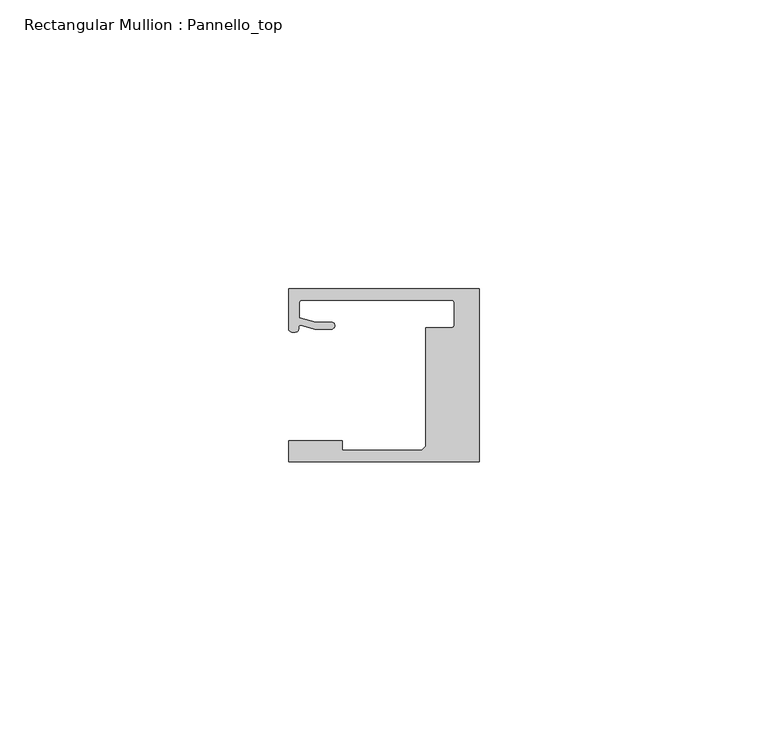
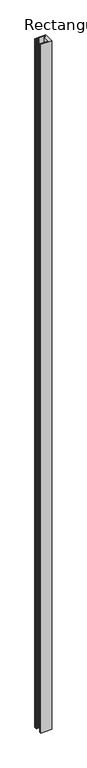
"""IFC4 building model written with IfcOpenShell, lengths in millimetres: member geometry, Rectangular Mullion : Pannello_top."""

from ifc_helpers import new_model, si_unit, frame, origin, place, context, project, spatial, polyline, circle_curve, source, transform, mapped, element, save
from ifc_brep_helpers import plane_surface, cylinder_surface, revolved_surface, extruded_surface, spline_curve, advanced_brep


def rectangular_mullion_pannello_top_90c1ebb8(model_context):
    return source(origin(), model_context, "Body", "AdvancedBrep", [
        advanced_brep(
        [(-33.0, -15.0, 0.0), (0.0, -15.0, 0.0), (0.0, 15.0, 0.0), (-33.0000135, 15.0, 0.0), (-33.0000135, 8.0000472, 0.0), (-30.9223017, 8.6490241, 0.0), (-28.4999305, 7.9999523, 0.0), (-25.59998, 7.9999523, 0.0), (-25.59998, 9.1999523, 0.0), (-28.3419477, 9.1999523, 0.0), (-31.19998, 9.9657591, 0.0), (-31.19998, 12.50001, 0.0), (-30.69998, 13.00001, 0.0), (-4.7999726, 13.00001, 0.0), (-4.2999726, 12.50001, 0.0), (-4.2999726, 8.7500595, 0.0), (-4.7999726, 8.2500595, 0.0), (-9.2999726, 8.2500595, 0.0), (-9.2999726, -12.2999849, 0.0), (-10.0000103, -13.0000004, 0.0), (-23.700041, -13.0000004, 0.0), (-23.700041, -11.3000004, 0.0), (-33.0, -11.3000004, 0.0), (-33.0, -15.0, -2173.9999729), (-33.0, -11.3000004, -2173.9999729), (-23.700041, -11.3000004, -2173.9999729), (-23.700041, -13.0000004, -2173.9999729), (-10.0000103, -13.0000004, -2173.9999729), (-9.2999726, -12.2999849, -2173.9999729), (-9.2999726, 8.2500595, -2173.9999729), (-4.7999726, 8.2500595, -2173.9999729), (-4.2999726, 8.7500595, -2173.9999729), (-4.2999726, 12.50001, -2173.9999729), (-4.7999726, 13.00001, -2173.9999729), (-30.69998, 13.00001, -2173.9999729), (-31.19998, 12.50001, -2173.9999729), (-31.19998, 9.9657591, -2173.9999729), (-28.3419477, 9.1999523, -2173.9999729), (-25.59998, 9.1999523, -2173.9999729), (-25.59998, 7.9999523, -2173.9999729), (-28.4999305, 7.9999523, -2173.9999729), (-30.9223017, 8.6490241, -2173.9999729), (-33.0000135, 8.0000472, -2173.9999729), (-33.0000135, 15.0, -2173.9999729), (0.0, 15.0, -2173.9999729), (0.0, -15.0, -2173.9999729)],
        [
            (0, 1),
            (1, 2),
            (2, 3),
            (3, 4),
            (4, 5, spline_curve(3, [(-33.0000135, 8.0000472, 0.0), (-33.0000135, 7.457047519, 0.0), (-32.262327879, 7.456527435, 0.0), (-31.357433266, 7.563996614, 0.0), (-31.305645054, 7.690065204, 0.0), (-31.298563602, 8.366228555, 0.0), (-31.312054066, 8.717747958, 0.0), (-30.9223017, 8.6490241, 0.0)], [4, 2, 2, 4], [0.0, 0.0027053965905959043, 0.0058611956533709, 0.007702013405570312])),
            (5, 6),
            (6, 7),
            (7, 8, circle_curve(frame((-25.59998, 8.5999523, 0.0), z_axis=(0.0, 0.0, 1.0), x_axis=(0.0, 1.0, 0.0)), 0.6)),
            (8, 9),
            (9, 10),
            (10, 11),
            (11, 12, circle_curve(frame((-30.69998, 12.50001, 0.0), z_axis=(0.0, 0.0, -1.0), x_axis=(0.0, 1.0, 0.0)), 0.5)),
            (12, 13),
            (13, 14, circle_curve(frame((-4.7999726, 12.50001, 0.0), z_axis=(0.0, 0.0, -1.0), x_axis=(1.0, 0.0, 0.0)), 0.5)),
            (14, 15),
            (15, 16, circle_curve(frame((-4.7999726, 8.7500595, 0.0), z_axis=(0.0, 0.0, -1.0), x_axis=(0.0, -1.0, 0.0)), 0.5)),
            (16, 17),
            (17, 18),
            (18, 19),
            (19, 20),
            (20, 21),
            (21, 22),
            (22, 0),
            (23, 24),
            (24, 25),
            (25, 26),
            (26, 27),
            (27, 28),
            (28, 29),
            (29, 30),
            (30, 31, circle_curve(frame((-4.7999726, 8.7500595, -2173.9999729), z_axis=(0.0, 0.0, 1.0), x_axis=(0.0, -1.0, 0.0)), 0.5)),
            (31, 32),
            (32, 33, circle_curve(frame((-4.7999726, 12.50001, -2173.9999729), z_axis=(0.0, 0.0, 1.0), x_axis=(1.0, 0.0, 0.0)), 0.5)),
            (33, 34),
            (34, 35, circle_curve(frame((-30.69998, 12.50001, -2173.9999729), z_axis=(0.0, 0.0, 1.0), x_axis=(0.0, 1.0, 0.0)), 0.5)),
            (35, 36),
            (36, 37),
            (37, 38),
            (38, 39, circle_curve(frame((-25.59998, 8.5999523, -2173.9999729), z_axis=(0.0, 0.0, -1.0), x_axis=(0.0, 1.0, 0.0)), 0.6)),
            (39, 40),
            (40, 41),
            (41, 42, spline_curve(3, [(-30.9223017, 8.6490241, -2173.9999729), (-31.312054066, 8.717747958, -2173.9999729), (-31.298563602, 8.366228555, -2173.9999729), (-31.305645054, 7.690065204, -2173.9999729), (-31.357433266, 7.563996614, -2173.9999729), (-32.262327879, 7.456527435, -2173.9999729), (-33.0000135, 7.457047519, -2173.9999729), (-33.0000135, 8.0000472, -2173.9999729)], [4, 2, 2, 4], [0.0, 0.001840817752199412, 0.004996616814974408, 0.007702013405570312])),
            (42, 43),
            (43, 44),
            (44, 45),
            (45, 23),
            (0, 23),
            (45, 1),
            (44, 2),
            (43, 3),
            (42, 4),
            (41, 5),
            (40, 6),
            (39, 7),
            (38, 8),
            (37, 9),
            (36, 10),
            (35, 11),
            (34, 12),
            (33, 13),
            (32, 14),
            (31, 15),
            (30, 16),
            (29, 17),
            (28, 18),
            (27, 19),
            (26, 20),
            (25, 21),
            (24, 22),
        ],
        [
            plane_surface(frame((0.0, -36.2491502, 0.0), z_axis=(0.0, 0.0, 1.0), x_axis=(-1.0, 0.0, 0.0))),
            plane_surface(frame((0.0, -36.2491502, -2173.9999729), z_axis=(0.0, 0.0, -1.0), x_axis=(-1.0, 0.0, 0.0))),
            plane_surface(frame((-33.0, -15.0, 0.0), z_axis=(0.0, -1.0, 0.0), x_axis=(0.0, 0.0, -1.0))),
            plane_surface(frame((0.0, -15.0, 0.0), z_axis=(1.0, 0.0, 0.0), x_axis=(0.0, 0.0, -1.0))),
            plane_surface(frame((0.0, 15.0, 0.0), z_axis=(0.0, 1.0, 0.0), x_axis=(0.0, 0.0, -1.0))),
            plane_surface(frame((-33.0000135, 15.0, 0.0), z_axis=(-1.0, 0.0, 0.0), x_axis=(0.0, 0.0, -1.0))),
            extruded_surface(spline_curve(3, [(-33.0000135, 8.0000472, -2173.9999729), (-33.0000135, 7.457047519, -2173.9999729), (-32.262327879, 7.456527435, -2173.9999729), (-31.357433266, 7.563996614, -2173.9999729), (-31.305645054, 7.690065204, -2173.9999729), (-31.298563602, 8.366228555, -2173.9999729), (-31.312054066, 8.717747958, -2173.9999729), (-30.9223017, 8.6490241, -2173.9999729)], [4, 2, 2, 4], [0.0, 0.0027053965905959043, 0.0058611956533709, 0.007702013405570312]), (0.0, 0.0, 2173.9999729), 2173.9999729),
            plane_surface(frame((-30.9223017, 8.6490241, 0.0), z_axis=(-0.25881883200192934, -0.9659258833891746, 0.0), x_axis=(0.0, 0.0, -1.0))),
            plane_surface(frame((-28.4999305, 7.9999523, 0.0), z_axis=(0.0, -1.0, 0.0), x_axis=(0.0, 0.0, -1.0))),
            cylinder_surface(frame((-25.59998, 8.5999523, 0.0), z_axis=(0.0, 0.0, 1.0), x_axis=(0.0, 1.0, 0.0)), 0.6),
            plane_surface(frame((-25.59998, 9.1999523, 0.0), z_axis=(0.0, 1.0, 0.0), x_axis=(0.0, 0.0, -1.0))),
            plane_surface(frame((-28.3419477, 9.1999523, 0.0), z_axis=(0.25881883204288636, 0.9659258833782002, 0.0), x_axis=(0.0, 0.0, -1.0))),
            plane_surface(frame((-31.19998, 9.9657591, 0.0), z_axis=(1.0, 0.0, 0.0), x_axis=(0.0, 0.0, -1.0))),
            revolved_surface(polyline([(-30.69998, 13.00001, -2173.9999729), (-30.69998, 13.00001, 0.0)]), (-30.69998, 12.50001, 0.0), (0.0, 0.0, -1.0)),
            plane_surface(frame((-30.69998, 13.00001, 0.0), z_axis=(0.0, -1.0, 0.0), x_axis=(0.0, 0.0, -1.0))),
            revolved_surface(polyline([(-4.2999726, 12.50001, -2173.9999729), (-4.2999726, 12.50001, 0.0)]), (-4.7999726, 12.50001, 0.0), (0.0, 0.0, -1.0)),
            plane_surface(frame((-4.2999726, 12.50001, 0.0), z_axis=(-1.0, 0.0, 0.0), x_axis=(0.0, 0.0, -1.0))),
            revolved_surface(polyline([(-4.7999726, 8.2500595, -2173.9999729), (-4.7999726, 8.2500595, 0.0)]), (-4.7999726, 8.7500595, 0.0), (0.0, 0.0, -1.0)),
            plane_surface(frame((-4.7999726, 8.2500595, 0.0), z_axis=(0.0, 1.0, 0.0), x_axis=(0.0, 0.0, -1.0))),
            plane_surface(frame((-9.2999726, 8.2500595, 0.0), z_axis=(-1.0, 0.0, 0.0), x_axis=(0.0, 0.0, -1.0))),
            plane_surface(frame((-9.2999726, -12.2999849, 0.0), z_axis=(-0.7070955486277984, 0.7071180135668678, 0.0), x_axis=(0.0, 0.0, -1.0))),
            plane_surface(frame((-10.0000103, -13.0000004, 0.0), z_axis=(0.0, 1.0, 0.0), x_axis=(0.0, 0.0, -1.0))),
            plane_surface(frame((-23.700041, -13.0000004, 0.0), z_axis=(1.0, 0.0, 0.0), x_axis=(0.0, 0.0, -1.0))),
            plane_surface(frame((-23.700041, -11.3000004, 0.0), z_axis=(0.0, 1.0, 0.0), x_axis=(0.0, 0.0, -1.0))),
            plane_surface(frame((-33.0, -11.3000004, 0.0), z_axis=(-1.0, 0.0, 0.0), x_axis=(0.0, 0.0, -1.0))),
        ],
        [
            (0, [[1, 2, 3, 4, 5, 6, 7, 8, 9, 10, 11, 12, 13, 14, 15, 16, 17, 18, 19, 20, 21, 22, 23]]),
            (1, [[24, 25, 26, 27, 28, 29, 30, 31, 32, 33, 34, 35, 36, 37, 38, 39, 40, 41, 42, 43, 44, 45, 46]]),
            (2, [[-1, 47, -46, 48]]),
            (3, [[-2, -48, -45, 49]]),
            (4, [[-3, -49, -44, 50]]),
            (5, [[-4, -50, -43, 51]]),
            (6, [[-5, -51, -42, 52]]),
            (7, [[-6, -52, -41, 53]]),
            (8, [[-7, -53, -40, 54]]),
            (9, [[-8, -54, -39, 55]]),
            (10, [[-9, -55, -38, 56]]),
            (11, [[-10, -56, -37, 57]]),
            (12, [[-11, -57, -36, 58]]),
            (13, [[-12, -58, -35, 59]]),
            (14, [[-13, -59, -34, 60]]),
            (15, [[-14, -60, -33, 61]]),
            (16, [[-15, -61, -32, 62]]),
            (17, [[-16, -62, -31, 63]]),
            (18, [[-17, -63, -30, 64]]),
            (19, [[-18, -64, -29, 65]]),
            (20, [[-19, -65, -28, 66]]),
            (21, [[-20, -66, -27, 67]]),
            (22, [[-21, -67, -26, 68]]),
            (23, [[-22, -68, -25, 69]]),
            (24, [[-23, -69, -24, -47]]),
        ],
    ),
    ])


if __name__ == "__main__":
    model = new_model("IFC4")
    model_context = context("Model", 3, world=origin())
    ifc_project = project(units=[si_unit("LENGTHUNIT", "METRE", prefix="MILLI")], contexts=[model_context])
    site = spatial("IfcSite", under=ifc_project)
    building = spatial("IfcBuilding", under=site)
    placement = place(None, origin())
    rectangular_mullion_pannello_top_shape = rectangular_mullion_pannello_top_90c1ebb8(model_context)
    element("IfcMember", 1, ObjectType="Rectangular Mullion : Pannello_top", at=placement, inside=building, context=model_context, shape_type="MappedRepresentation", body=[
        mapped(rectangular_mullion_pannello_top_shape, transform((0.0, 0.0, 0.0), x_axis=(1.0, 0.0, 0.0), y_axis=(0.0, 1.0, 0.0), z_axis=(0.0, 0.0, 1.0))),
    ])
    save(model, "model.ifc")

# Revit data of these elements
# Type "Rectangular Mullion : Pannello_top"
#   built-in parameter 1007322 = 0.0984252 (stored number, unit not read)
#   built-in parameter 1007321 = 0 (stored number, unit not read)
#   built-in parameter 1007320 = 0.0305117 (stored number, unit not read)
